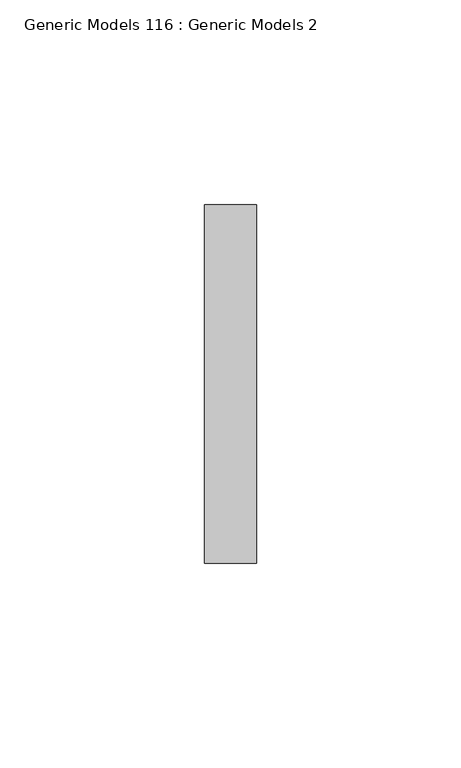
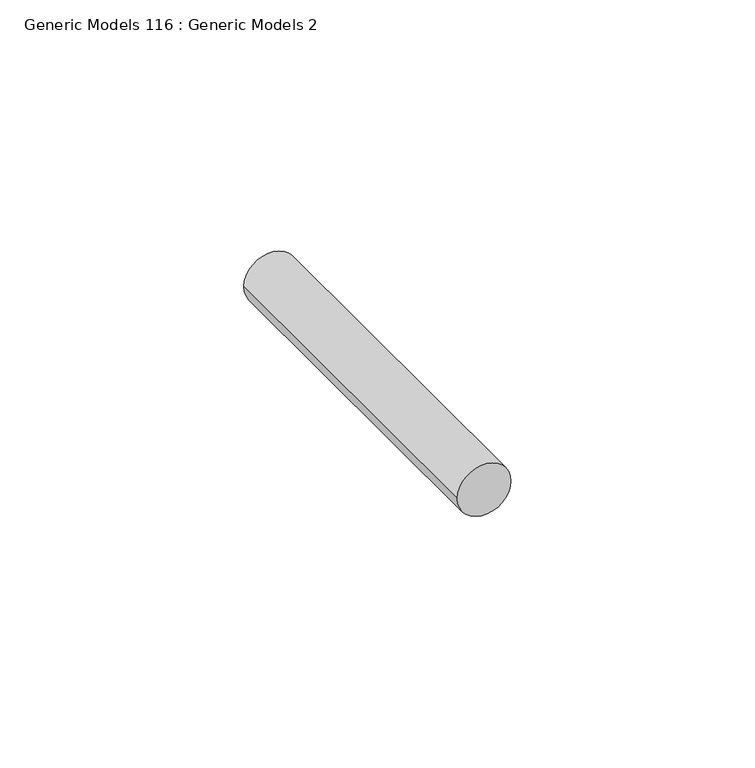
"""IFC4 building model written with IfcOpenShell, lengths in millimetres: proxy geometry, Generic Models 116 : Generic Models 2."""

from ifc_helpers import new_model, si_unit, point, frame, frame_2d, origin, place, context, project, spatial, circle_curve, trimmed, segment, composite_curve, outline, extrude, source, transform, mapped, element, save


def generic_models_116_generic_models_2_f9cbcbe1(model_context):
    return source(origin(), model_context, "Body", "SweptSolid", [
        extrude(outline(composite_curve([segment(trimmed(circle_curve(frame_2d((37860.4162436, 6738.7346014)), 6.35), [point((37860.4162436, 6745.0846014))], [point((37860.4162436, 6732.3846014))], False, "CARTESIAN"), True, "CONTINUOUS"), segment(trimmed(circle_curve(frame_2d((37860.4162436, 6738.7346014)), 6.35), [point((37860.4162436, 6732.3846014))], [point((37860.4162436, 6745.0846014))], False, "CARTESIAN"), True, "CONTINUOUS")], self_intersect=False)), frame((0.0, 1848.3666731, 0.0), z_axis=(0.0, 1.0, 0.0), x_axis=(0.0, 0.0, 1.0)), (0.0, 0.0, 1.0), 87.551022),
    ])


if __name__ == "__main__":
    model = new_model("IFC4")
    model_context = context("Model", 3, world=origin())
    ifc_project = project(units=[si_unit("LENGTHUNIT", "METRE", prefix="MILLI")], contexts=[model_context])
    site = spatial("IfcSite", under=ifc_project)
    building = spatial("IfcBuilding", under=site)
    placement = place(None, origin())
    generic_models_116_generic_models_2_shape = generic_models_116_generic_models_2_f9cbcbe1(model_context)
    element("IfcBuildingElementProxy", 1, Name="Generic Models 116 : Generic Models 2", ObjectType="Generic Models 116 : Generic Models 2", at=placement, inside=building, context=model_context, shape_type="MappedRepresentation", body=[
        mapped(generic_models_116_generic_models_2_shape, transform((0.0, 0.0, 0.0), x_axis=(1.0, 0.0, 0.0), y_axis=(0.0, 1.0, 0.0), z_axis=(0.0, 0.0, 1.0))),
    ])
    save(model, "model.ifc")

# Revit data of these elements
# Element 1 (IfcBuildingElementProxy, "Generic Models 116 : Generic Models 2")
#   Materials on its faces: "S.S. LAG BOLT - SEE STRUCT. DWGS"
# Materials
#   "S.S. LAG BOLT - SEE STRUCT. DWGS": class "Generic", colour RGB 120 120 120, transparency 0, Cost = 0
